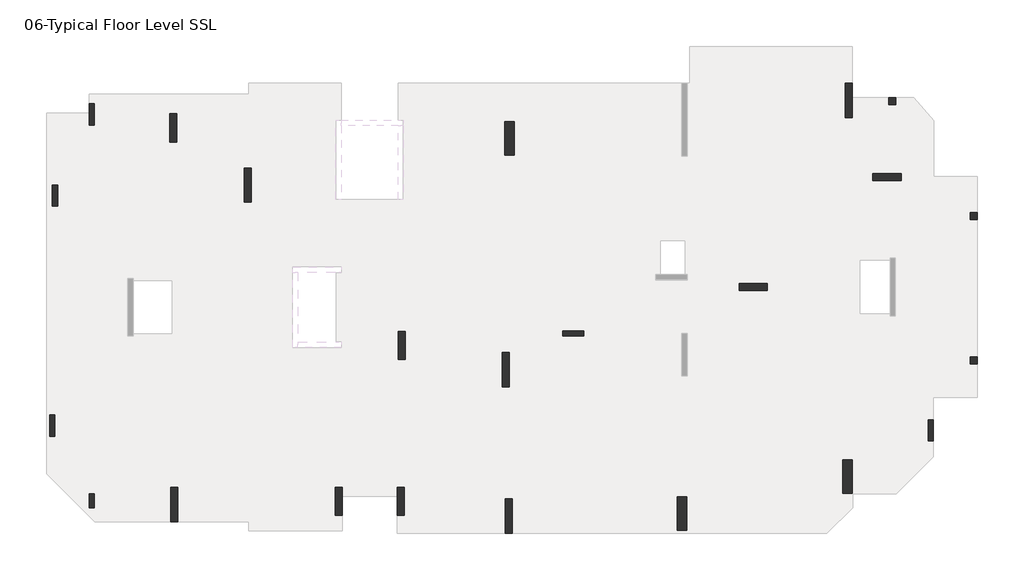
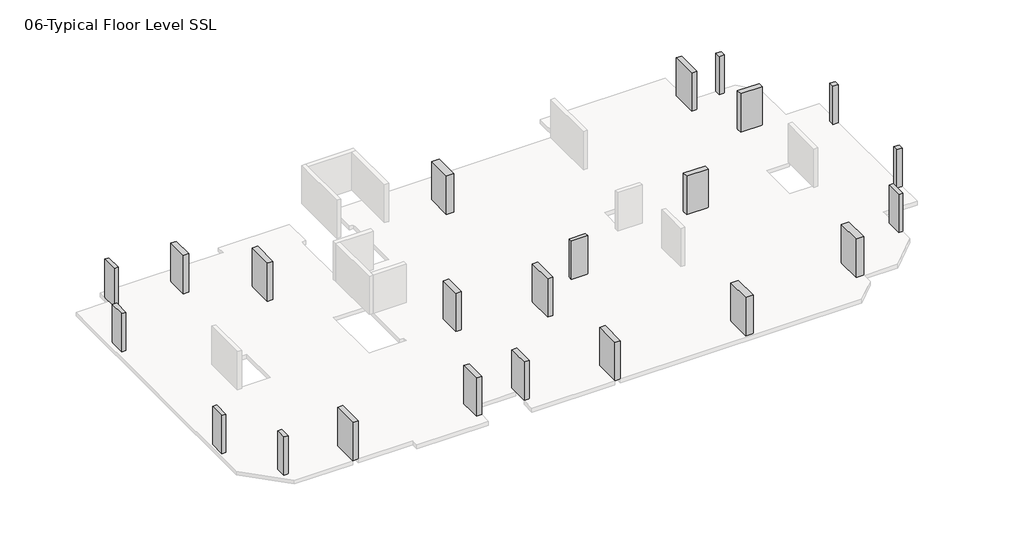
# One storey, part 2 of 2: 23 columns.
"""IFC4 building model written with IfcOpenShell, lengths in millimetres."""

import ifcopenshell
import ifcopenshell.guid

model = None  # the IFC model being written
_history = None  # IfcOwnerHistory: only IFC2X3 demands one
_inside = {}  # id of a spatial element -> (the spatial element, [elements in it])
_under = {}  # id of a project, library or spatial element -> (it, [spatial elements below it])
_declared = {}  # id of a project -> (the project, [libraries it declares])
_typed = {}  # id of a type object -> (the type object, [elements of that type])
_made_of = {}  # id of a material, layer set ... -> (it, [elements and type objects made of it])


def new_model(schema):
    """Start an empty IFC model of exactly this schema.

    Asked for "IFC4X3", IfcOpenShell would pick the latest addendum, in which some entities
    have other attributes; the version numbers below select the first issue.
    IFC2X3 requires an IfcOwnerHistory on every rooted entity: one is made here for all.
    """
    global model, _history
    if schema == "IFC4X3":
        model = ifcopenshell.file(schema_version=(4, 3, 0, 0))
    else:
        model = ifcopenshell.file(schema=schema)
    _inside.clear()
    _under.clear()
    _declared.clear()
    _typed.clear()
    _made_of.clear()
    _history = None
    if model.schema == "IFC2X3":
        org = make("IfcOrganization", Name="unknown")
        user = make(
            "IfcPersonAndOrganization",
            ThePerson=make("IfcPerson", FamilyName="unknown"),
            TheOrganization=org,
        )
        app = make(
            "IfcApplication",
            ApplicationDeveloper=org,
            Version="unknown",
            ApplicationFullName="unknown",
            ApplicationIdentifier="unknown",
        )
        _history = make(
            "IfcOwnerHistory",
            OwningUser=user,
            OwningApplication=app,
            ChangeAction="ADDED",
            CreationDate=0,
        )
    return model


def make(cls, **values):
    """One entity of the class cls with the attributes given. An attribute that is None is left unset."""
    return model.create_entity(
        cls, **{name: value for name, value in values.items() if value is not None}
    )


def rooted(cls, **values):
    """An entity with a GlobalId (a new one), such as an element, a storey or a relation."""
    return make(cls, GlobalId=ifcopenshell.guid.new(), OwnerHistory=_history, **values)


def si_unit(unit_type, name, prefix=None):
    """IfcSIUnit, for example si_unit("LENGTHUNIT", "METRE", prefix="MILLI")."""
    return make("IfcSIUnit", UnitType=unit_type, Prefix=prefix, Name=name)


def assignment(units):
    """IfcUnitAssignment: the units of a project."""
    return None if units is None else make("IfcUnitAssignment", Units=units)


def point(xyz):
    """IfcCartesianPoint."""
    return None if xyz is None else make("IfcCartesianPoint", Coordinates=xyz)


def direction(xyz):
    """IfcDirection."""
    return None if xyz is None else make("IfcDirection", DirectionRatios=xyz)


def frame(location, z_axis=None, x_axis=None):
    """IfcAxis2Placement3D, a coordinate frame: its origin and axes. An axis left out is left unset."""
    return make(
        "IfcAxis2Placement3D",
        Location=point(location),
        Axis=direction(z_axis),
        RefDirection=direction(x_axis),
    )


def origin():
    """The frame at (0, 0, 0) with its axes left unset."""
    return frame((0.0, 0.0, 0.0))


def place(relative_to, where):
    """IfcLocalPlacement: puts the frame where relative to a parent placement (None: the world)."""
    return make(
        "IfcLocalPlacement", PlacementRelTo=relative_to, RelativePlacement=where
    )


def context(
    kind, dimensions, precision=None, world=None, true_north=None, identifier=None
):
    """IfcGeometricRepresentationContext, for example the 3D "Model" context."""
    return make(
        "IfcGeometricRepresentationContext",
        ContextIdentifier=identifier,
        ContextType=kind,
        CoordinateSpaceDimension=dimensions,
        Precision=precision,
        WorldCoordinateSystem=world,
        TrueNorth=true_north,
    )


def project(units=None, contexts=None):
    """IfcProject with its units and contexts."""
    return rooted(
        "IfcProject",
        Name="project",
        RepresentationContexts=contexts,
        UnitsInContext=assignment(units),
    )


def spatial(cls, under=None, at=None, **own):
    """A site, building, storey or space (cls), placed at a placement, below another one or the project."""
    s = rooted(cls, ObjectPlacement=at, **own)
    if under is not None:
        _under.setdefault(under.id(), (under, []))[1].append(s)
    return s


def faces_of(points, faces, orient=None, outer=None):
    """IfcFace entities. A face is a list of loops; a loop is a list of indices into points, from 0.

    orient and outer hold one flag for each loop. By default every Orientation is true, the
    first loop of a face is its IfcFaceOuterBound and the others are IfcFaceBound.
    """
    made = []
    for i, loops in enumerate(faces):
        bounds = []
        for j, loop in enumerate(loops):
            is_outer = j == 0 if outer is None else outer[i][j]
            bounds.append(
                make(
                    "IfcFaceOuterBound" if is_outer else "IfcFaceBound",
                    Bound=make("IfcPolyLoop", Polygon=[points[k] for k in loop]),
                    Orientation=True if orient is None else orient[i][j],
                )
            )
        made.append(make("IfcFace", Bounds=bounds))
    return made


def faceted_brep(points, faces, orient=None, outer=None, voids=None):
    """IfcFacetedBrep: a solid bounded by flat faces; with voids (closed shells), ...WithVoids."""
    shared = [point(p) for p in points]
    hull = make("IfcClosedShell", CfsFaces=faces_of(shared, faces, orient, outer))
    if voids is None:
        return make("IfcFacetedBrep", Outer=hull)
    return make(
        "IfcFacetedBrepWithVoids",
        Outer=hull,
        Voids=[
            make(cls, CfsFaces=faces_of(shared, fs, o, b)) for cls, fs, o, b in voids
        ],
    )


def shape(context_of_items, identifier, shape_type, items):
    """IfcShapeRepresentation: the items that make up one representation, for example the "Body"."""
    return make(
        "IfcShapeRepresentation",
        ContextOfItems=context_of_items,
        RepresentationIdentifier=identifier,
        RepresentationType=shape_type,
        Items=items,
    )


def made_of(thing, what):
    """Note that an element or type object is made of a material, layer set ...; save() writes the relation."""
    if what is not None:
        _made_of.setdefault(what.id(), (what, []))[1].append(thing)
    return thing


def element(
    cls,
    number,
    at=None,
    inside=None,
    cuts=None,
    type_object=None,
    material=None,
    context=None,
    identifier="Body",
    shape_type=None,
    held_by="IfcProductDefinitionShape",
    body=None,
    shapes=None,
    **own,
):
    """One element of the class cls, such as IfcWall. Its Tag is "e" and its number.

    at: its placement. inside: the storey or other place that contains it. cuts: it is an
    opening in that element (IfcRelVoidsElement). A single representation is given by context,
    identifier, shape_type and body (its items); several are given by shapes. held_by: the class
    of the entity that holds the representations. save() writes the other relations.
    """
    e = rooted(cls, Tag="e%d" % number, ObjectPlacement=at, **own)
    if body is not None:
        shapes = [shape(context, identifier, shape_type, body)]
    if shapes is not None:
        e.Representation = make(held_by, Representations=shapes)
    if inside is not None:
        _inside.setdefault(inside.id(), (inside, []))[1].append(e)
    if cuts is not None:
        rooted(
            "IfcRelVoidsElement", RelatingBuildingElement=cuts, RelatedOpeningElement=e
        )
    if type_object is not None:
        _typed.setdefault(type_object.id(), (type_object, []))[1].append(e)
    return made_of(e, material)


def aggregate(whole, parts):
    """IfcRelAggregates: a whole, such as a stair, and the parts it consists of."""
    return rooted("IfcRelAggregates", RelatingObject=whole, RelatedObjects=parts)


def save(model, path):
    """Write the relations noted so far, then the file.

    IfcRelAggregates (storeys below a building ...), IfcRelContainedInSpatialStructure (elements
    in a storey), IfcRelDefinesByType, IfcRelAssociatesMaterial and IfcRelDeclares: one each for
    every whole, place, type object, material and project.
    """
    for whole, parts in _under.values():
        aggregate(whole, parts)
    for where, things in _inside.values():
        rooted(
            "IfcRelContainedInSpatialStructure",
            RelatedElements=things,
            RelatingStructure=where,
        )
    for kind, things in _typed.values():
        rooted("IfcRelDefinesByType", RelatedObjects=things, RelatingType=kind)
    for what, things in _made_of.values():
        rooted("IfcRelAssociatesMaterial", RelatedObjects=things, RelatingMaterial=what)
    for by, libraries in _declared.values():
        rooted("IfcRelDeclares", RelatingContext=by, RelatedDefinitions=libraries)
    model.write(path)


model = new_model("IFC4")

# Units and contexts
model_context = context("Model", 3, world=origin())
ifc_project = project(units=[si_unit("LENGTHUNIT", "METRE", prefix="MILLI")], contexts=[model_context])

# Site, building, storey
site = spatial("IfcSite", under=ifc_project)
building = spatial("IfcBuilding", under=site)
storey = spatial("IfcBuildingStorey", under=building, Name="06-Typical Floor Level SSL", Elevation=12000.0)

# Columns
placement = place(None, origin())
element("IfcColumn", 1, ObjectType="M_Concrete-Rectangular-Column : C-1 (400 x 400mm)", at=placement, inside=storey, context=model_context, shape_type="Brep", body=[
    faceted_brep([(52549.9999998, 16712.0, 12000.0), (52549.9999998, 16312.0, 12000.0), (52149.9999998, 16312.0, 12000.0), (52149.9999998, 16712.0, 12000.0), (52549.9999998, 16712.0, 15000.0), (52549.9999998, 16312.0, 15000.0), (52549.9999998, 16312.0, 14700.0), (52549.9999998, 16712.0, 14700.0), (52149.9999998, 16312.0, 15000.0), (52149.9999998, 16312.0, 14700.0), (52149.9999998, 16712.0, 15000.0), (52149.9999998, 16712.0, 14700.0)], [[[0, 1, 2, 3]], [[4, 5, 6, 1, 0, 7]], [[5, 8, 9, 2, 1, 6]], [[8, 10, 11, 3, 2, 9]], [[10, 4, 7, 0, 3, 11]], [[4, 10, 8, 5]]]),
])
element("IfcColumn", 2, ObjectType="M_Concrete-Rectangular-Column : C-1 (400 x 400mm)", at=placement, inside=storey, context=model_context, shape_type="Brep", body=[
    faceted_brep([(47898.6337868, 23252.0, 12000.0), (47898.6337868, 22852.0, 12000.0), (47498.6337868, 22852.0, 12000.0), (47498.6337868, 23252.0, 12000.0), (47898.6337868, 23252.0, 15000.0), (47898.6337868, 22852.0, 15000.0), (47898.6337868, 22852.0, 14700.0), (47498.6337868, 22852.0, 15000.0), (47498.6337868, 22852.0, 14700.0), (47498.6337868, 23252.0, 15000.0)], [[[0, 1, 2, 3]], [[4, 5, 6, 1, 0]], [[5, 7, 8, 2, 1, 6]], [[7, 9, 3, 2, 8]], [[9, 4, 0, 3]], [[4, 9, 7, 5]]]),
])
element("IfcColumn", 3, ObjectType="M_Concrete-Rectangular-Column : C-1 (400 x 400mm)", at=placement, inside=storey, context=model_context, shape_type="Brep", body=[
    faceted_brep([(52549.9999998, 8504.0039609, 12000.0), (52549.9999998, 8104.0039609, 12000.0), (52149.9999998, 8104.0039609, 12000.0), (52149.9999998, 8504.0039609, 12000.0), (52549.9999998, 8504.0039609, 15000.0), (52549.9999998, 8104.0039609, 15000.0), (52549.9999998, 8104.0039609, 14700.0), (52549.9999998, 8504.0039609, 14700.0), (52149.9999998, 8104.0039609, 15000.0), (52149.9999998, 8104.0039609, 14700.0), (52149.9999998, 8504.0039609, 15000.0), (52149.9999998, 8504.0039609, 14700.0)], [[[0, 1, 2, 3]], [[4, 5, 6, 1, 0, 7]], [[5, 8, 9, 2, 1, 6]], [[8, 10, 11, 3, 2, 9]], [[10, 4, 7, 0, 3, 11]], [[4, 10, 8, 5]]]),
])
element("IfcColumn", 4, ObjectType="M_Concrete-Rectangular-Column : C-2 (300 x 800mm)", at=placement, inside=storey, context=model_context, shape_type="Brep", body=[
    faceted_brep([(2352.0, 728.0, 12000.0), (2352.0, -72.0, 12000.0), (2052.0, -72.0, 12000.0), (2052.0, 728.0, 12000.0), (2352.0, 728.0, 15000.0), (2352.0, -72.0, 15000.0), (2352.0, -72.0, 14700.0), (2352.0, 728.0, 14700.0), (2052.0, -72.0, 15000.0), (2052.0, -72.0, 14700.0), (2052.0, 728.0, 15000.0), (2052.0, 728.0, 14700.0)], [[[0, 1, 2, 3]], [[4, 5, 6, 1, 0, 7]], [[5, 8, 9, 2, 1, 6]], [[8, 10, 11, 3, 2, 9]], [[10, 4, 7, 0, 3, 11]], [[4, 10, 8, 5]]]),
])
element("IfcColumn", 5, ObjectType="M_Concrete-Rectangular-Column : C-3(300 x 1200mm)", at=placement, inside=storey, context=model_context, shape_type="Brep", body=[
    faceted_brep([(2352.0, 22908.0000656, 12000.0), (2352.0, 21708.0000656, 12000.0), (2052.0, 21708.0000656, 12000.0), (2052.0, 22908.0000656, 12000.0), (2352.0, 22908.0000656, 15000.0), (2352.0, 21708.0000656, 15000.0), (2352.0, 21708.0000656, 14700.0), (2352.0, 22908.0000656, 14700.0), (2052.0, 21708.0000656, 15000.0), (2052.0, 21708.0000656, 14700.0), (2052.0, 22380.0004589, 15000.0), (2052.0, 22908.0000656, 15000.0), (2052.0, 22908.0000656, 14700.0)], [[[0, 1, 2, 3]], [[4, 5, 6, 1, 0, 7]], [[5, 8, 9, 2, 1, 6]], [[8, 10, 11, 12, 3, 2, 9]], [[11, 4, 7, 0, 3, 12]], [[4, 11, 10, 8, 5]]]),
])
element("IfcColumn", 6, ObjectType="M_Concrete-Rectangular-Column : C-3(300 x 1200mm)", at=placement, inside=storey, context=model_context, shape_type="Brep", body=[
    faceted_brep([(257.9999999, 18288.0, 12000.0), (257.9999999, 17088.0, 12000.0), (-42.0000001, 17088.0, 12000.0), (-42.0000001, 18288.0, 12000.0), (257.9999999, 18288.0, 15000.0), (257.9999999, 17088.0, 15000.0), (257.9999999, 17088.0, 14700.0), (257.9999999, 18288.0, 14700.0), (-42.0000001, 17088.0, 15000.0), (-42.0000001, 17088.0, 14700.0), (-42.0000001, 18288.0, 15000.0), (-42.0000001, 18288.0, 14700.0)], [[[0, 1, 2, 3]], [[4, 5, 6, 1, 0, 7]], [[5, 8, 9, 2, 1, 6]], [[8, 10, 11, 3, 2, 9]], [[10, 4, 7, 0, 3, 11]], [[4, 10, 8, 5]]]),
])
element("IfcColumn", 7, ObjectType="M_Concrete-Rectangular-Column : C-3(300 x 1200mm)", at=placement, inside=storey, context=model_context, shape_type="Brep", body=[
    faceted_brep([(108.001803, 5201.9999858, 12000.0), (108.001803, 4001.9999858, 12000.0), (-191.998197, 4001.9999858, 12000.0), (-191.998197, 5201.9999858, 12000.0), (108.001803, 5201.9999858, 15000.0), (108.001803, 4001.9999858, 15000.0), (108.001803, 4001.9999858, 14700.0), (108.001803, 5201.9999858, 14700.0), (-191.998197, 4001.9999858, 15000.0), (-191.998197, 4001.9999858, 14700.0), (-191.998197, 5201.9999858, 15000.0), (-191.998197, 5201.9999858, 14700.0)], [[[0, 1, 2, 3]], [[4, 5, 6, 1, 0, 7]], [[5, 8, 9, 2, 1, 6]], [[8, 10, 11, 3, 2, 9]], [[10, 4, 7, 0, 3, 11]], [[4, 10, 8, 5]]]),
])
element("IfcColumn", 8, ObjectType="M_Concrete-Rectangular-Column : C-3(300 x 1200mm)", at=placement, inside=storey, context=model_context, shape_type="Brep", body=[
    faceted_brep([(50046.0009271, 4931.9999929, 12000.0), (50046.0009271, 3731.9999929, 12000.0), (49746.0009271, 3731.9999929, 12000.0), (49746.0009271, 4931.9999929, 12000.0), (50046.0009271, 4931.9999929, 15000.0), (50046.0009271, 3731.9999929, 15000.0), (50046.0009271, 3731.9999929, 14700.0), (50046.0009271, 4931.9999929, 14700.0), (49746.0009271, 3731.9999929, 15000.0), (49746.0009271, 3731.9999929, 14700.0), (49746.0009271, 4931.9999929, 15000.0), (49746.0009271, 4931.9999929, 14700.0)], [[[0, 1, 2, 3]], [[4, 5, 6, 1, 0, 7]], [[5, 8, 9, 2, 1, 6]], [[8, 10, 11, 3, 2, 9]], [[10, 4, 7, 0, 3, 11]], [[4, 10, 8, 5]]]),
])
element("IfcColumn", 9, ObjectType="M_Concrete-Rectangular-Column : C-3(300 x 1200mm)", at=placement, inside=storey, context=model_context, shape_type="Brep", body=[
    faceted_brep([(28975.9999998, 9996.0000019, 12000.0), (30175.9999998, 9996.0000019, 12000.0), (30175.9999998, 9696.0000019, 12000.0), (28975.9999998, 9696.0000019, 12000.0), (28975.9999998, 9996.0000019, 15000.0), (30175.9999998, 9996.0000019, 15000.0), (30175.9999998, 9996.0000019, 14700.0), (28975.9999998, 9996.0000019, 14700.0), (30175.9999998, 9696.0000019, 15000.0), (30175.9999998, 9696.0000019, 14700.0), (28975.9999998, 9696.0000019, 15000.0), (28975.9999998, 9696.0000019, 14700.0)], [[[0, 1, 2, 3]], [[4, 5, 6, 1, 0, 7]], [[5, 8, 9, 2, 1, 6]], [[8, 10, 11, 3, 2, 9]], [[10, 4, 7, 0, 3, 11]], [[4, 10, 8, 5]]]),
])
element("IfcColumn", 10, ObjectType="M_Concrete-Rectangular-Column : C-4 (400 x 1600mm)", at=placement, inside=storey, context=model_context, shape_type="Brep", body=[
    faceted_brep([(7021.9999999, 22340.0000078, 12000.0), (7021.9999999, 20740.0000078, 12000.0), (6621.9999999, 20740.0000078, 12000.0), (6621.9999999, 22340.0000078, 12000.0), (7021.9999999, 22340.0000078, 15000.0), (7021.9999999, 20740.0000078, 15000.0), (7021.9999999, 20740.0000078, 14700.0), (7021.9999999, 22340.0000078, 14700.0), (6621.9999999, 20740.0000078, 15000.0), (6621.9999999, 20740.0000078, 14700.0), (6621.9999999, 22340.0000078, 15000.0), (6621.9999999, 22340.0000078, 14700.0)], [[[0, 1, 2, 3]], [[4, 5, 6, 1, 0, 7]], [[5, 8, 9, 2, 1, 6]], [[8, 10, 11, 3, 2, 9]], [[10, 4, 7, 0, 3, 11]], [[4, 10, 8, 5]]]),
])
element("IfcColumn", 11, ObjectType="M_Concrete-Rectangular-Column : C-4 (400 x 1600mm)", at=placement, inside=storey, context=model_context, shape_type="Brep", body=[
    faceted_brep([(19969.9997488, 1087.9955348, 12000.0), (19969.9997488, -512.0044652, 12000.0), (19569.9997488, -512.0044652, 12000.0), (19569.9997488, 1087.9955348, 12000.0), (19969.9997488, 1087.9955348, 15000.0), (19969.9997488, -512.0044652, 15000.0), (19969.9997488, -512.0044652, 14700.0), (19969.9997488, 1087.9955348, 14700.0), (19569.9997488, -512.0044652, 15000.0), (19569.9997488, -512.0044652, 14700.0), (19569.9997488, 564.000519, 15000.0), (19569.9997488, 1087.9955348, 15000.0), (19569.9997488, 1087.9955348, 14700.0)], [[[0, 1, 2, 3]], [[4, 5, 6, 1, 0, 7]], [[5, 8, 9, 2, 1, 6]], [[8, 10, 11, 12, 3, 2, 9]], [[11, 4, 7, 0, 3, 12]], [[4, 11, 10, 8, 5]]]),
])
element("IfcColumn", 12, ObjectType="M_Concrete-Rectangular-Column : C-4 (400 x 1600mm)", at=placement, inside=storey, context=model_context, shape_type="Brep", body=[
    faceted_brep([(46605.9993605, 18950.0, 12000.0), (48205.9993605, 18950.0, 12000.0), (48205.9993605, 18550.0, 12000.0), (46605.9993605, 18550.0, 12000.0), (46605.9993605, 18950.0, 15000.0), (48205.9993605, 18950.0, 15000.0), (48205.9993605, 18950.0, 14700.0), (46605.9993605, 18950.0, 14700.0), (48205.9993605, 18550.0, 15000.0), (48205.9993605, 18550.0, 14700.0), (46605.9993605, 18550.0, 15000.0), (46605.9993605, 18550.0, 14700.0)], [[[0, 1, 2, 3]], [[4, 5, 6, 1, 0, 7]], [[5, 8, 9, 2, 1, 6]], [[8, 10, 11, 3, 2, 9]], [[10, 4, 7, 0, 3, 11]], [[4, 10, 8, 5]]]),
])
element("IfcColumn", 13, ObjectType="M_Concrete-Rectangular-Column : C-5 (400 x 1600mm)", at=placement, inside=storey, context=model_context, shape_type="Brep", body=[
    faceted_brep([(20030.000009, 9955.9999979, 12000.0), (20030.000009, 8355.9999979, 12000.0), (19630.000009, 8355.9999979, 12000.0), (19630.000009, 9955.9999979, 12000.0), (20030.000009, 9955.9999979, 15000.0), (20030.000009, 8355.9999979, 15000.0), (20030.000009, 8355.9999979, 14700.0), (20030.000009, 9955.9999979, 14700.0), (19630.000009, 8355.9999979, 15000.0), (19630.000009, 8355.9999979, 14700.0), (19630.000009, 9955.9999979, 15000.0), (19630.000009, 9955.9999979, 14700.0)], [[[0, 1, 2, 3]], [[4, 5, 6, 1, 0, 7]], [[5, 8, 9, 2, 1, 6]], [[8, 10, 11, 3, 2, 9]], [[10, 4, 7, 0, 3, 11]], [[4, 10, 8, 5]]]),
])
element("IfcColumn", 14, ObjectType="M_Concrete-Rectangular-Column : C-5 (400 x 1600mm)", at=placement, inside=storey, context=model_context, shape_type="Brep", body=[
    faceted_brep([(16429.9999981, 1088.0, 12000.0), (16429.9999981, -512.0, 12000.0), (16029.9999981, -512.0, 12000.0), (16029.9999981, 1088.0, 12000.0), (16429.9999981, 1088.0, 15000.0), (16429.9999981, 564.000519, 15000.0), (16429.9999981, -512.0, 15000.0), (16429.9999981, -512.0, 14700.0), (16429.9999981, 1088.0, 14700.0), (16029.9999981, -512.0, 15000.0), (16029.9999981, -512.0, 14700.0), (16029.9999981, 1088.0, 15000.0), (16029.9999981, 1088.0, 14700.0)], [[[0, 1, 2, 3]], [[4, 5, 6, 7, 1, 0, 8]], [[6, 9, 10, 2, 1, 7]], [[9, 11, 12, 3, 2, 10]], [[11, 4, 8, 0, 3, 12]], [[4, 11, 9, 6, 5]]]),
])
element("IfcColumn", 15, ObjectType="M_Concrete-Rectangular-Column : C-5 (400 x 1600mm)", at=placement, inside=storey, context=model_context, shape_type="Brep", body=[
    faceted_brep([(38998.0014887, 12692.0079212, 12000.0), (40598.0014887, 12692.0079212, 12000.0), (40598.0014887, 12292.0079212, 12000.0), (38998.0014887, 12292.0079212, 12000.0), (38998.0014887, 12692.0079212, 15000.0), (40598.0014887, 12692.0079212, 15000.0), (40598.0014887, 12692.0079212, 14700.0), (38998.0014887, 12692.0079212, 14700.0), (40598.0014887, 12292.0079212, 15000.0), (40598.0014887, 12292.0079212, 14700.0), (38998.0014887, 12292.0079212, 15000.0), (38998.0014887, 12292.0079212, 14700.0)], [[[0, 1, 2, 3]], [[4, 5, 6, 1, 0, 7]], [[5, 8, 9, 2, 1, 6]], [[8, 10, 11, 3, 2, 9]], [[10, 4, 7, 0, 3, 11]], [[4, 10, 8, 5]]]),
])
element("IfcColumn", 16, ObjectType="M_Concrete-Rectangular-Column : C-6 (400 x 1950mm)", at=placement, inside=storey, context=model_context, shape_type="Brep", body=[
    faceted_brep([(11270.0000427, 19262.9999996, 12000.0), (11270.0000427, 17312.9999996, 12000.0), (10870.0000427, 17312.9999996, 12000.0), (10870.0000427, 19262.9999996, 12000.0), (11270.0000427, 19262.9999996, 15000.0), (11270.0000427, 17312.9999996, 15000.0), (11270.0000427, 17312.9999996, 14700.0), (11270.0000427, 19262.9999996, 14700.0), (10870.0000427, 17312.9999996, 15000.0), (10870.0000427, 17312.9999996, 14700.0), (10870.0000427, 19262.9999996, 15000.0), (10870.0000427, 19262.9999996, 14700.0)], [[[0, 1, 2, 3]], [[4, 5, 6, 1, 0, 7]], [[5, 8, 9, 2, 1, 6]], [[8, 10, 11, 3, 2, 9]], [[10, 4, 7, 0, 3, 11]], [[4, 10, 8, 5]]]),
])
element("IfcColumn", 17, ObjectType="M_Concrete-Rectangular-Column : C-6 (400 x 1950mm)", at=placement, inside=storey, context=model_context, shape_type="Brep", body=[
    faceted_brep([(7082.0000416, 1083.0000153, 12000.0), (7082.0000416, -866.9999847, 12000.0), (6682.0000416, -866.9999847, 12000.0), (6682.0000416, 1083.0000153, 12000.0), (7082.0000416, 1083.0000153, 15000.0), (7082.0000416, -866.9999847, 15000.0), (7082.0000416, -866.9999847, 14700.0), (7082.0000416, 1083.0000153, 14700.0), (6682.0000416, -866.9999847, 15000.0), (6682.0000416, -866.9999847, 14700.0), (6682.0000416, 1083.0000153, 15000.0), (6682.0000416, 1083.0000153, 14700.0)], [[[0, 1, 2, 3]], [[4, 5, 6, 1, 0, 7]], [[5, 8, 9, 2, 1, 6]], [[8, 10, 11, 3, 2, 9]], [[10, 4, 7, 0, 3, 11]], [[4, 10, 8, 5]]]),
])
element("IfcColumn", 18, ObjectType="M_Concrete-Rectangular-Column : C-6 (400 x 1950mm)", at=placement, inside=storey, context=model_context, shape_type="Brep", body=[
    faceted_brep([(26113.9999998, 422.995535, 12000.0), (26113.9999998, -1527.004465, 12000.0), (25713.9999998, -1527.004465, 12000.0), (25713.9999998, 422.995535, 12000.0), (26113.9999998, 422.995535, 15000.0), (26113.9999998, -1527.004465, 15000.0), (26113.9999998, -1527.004465, 14700.0), (26113.9999998, 422.995535, 14700.0), (25713.9999998, -1527.004465, 15000.0), (25713.9999998, -1527.004465, 14700.0), (25713.9999998, 422.995535, 15000.0), (25713.9999998, 422.995535, 14700.0)], [[[0, 1, 2, 3]], [[4, 5, 6, 1, 0, 7]], [[5, 8, 9, 2, 1, 6]], [[8, 10, 11, 3, 2, 9]], [[10, 4, 7, 0, 3, 11]], [[4, 10, 8, 5]]]),
])
element("IfcColumn", 19, ObjectType="M_Concrete-Rectangular-Column : C-6 (400 x 1950mm)", at=placement, inside=storey, context=model_context, shape_type="Brep", body=[
    faceted_brep([(45446.0007483, 24087.0, 12000.0), (45446.0007483, 22137.0, 12000.0), (45046.0007483, 22137.0, 12000.0), (45046.0007483, 24087.0, 12000.0), (45446.0007483, 24087.0, 15000.0), (45446.0007483, 23252.0000315, 15000.0), (45446.0007483, 22137.0, 15000.0), (45446.0007483, 22137.0, 14700.0), (45446.0007483, 24087.0, 14700.0), (45046.0007483, 22137.0, 15000.0), (45046.0007483, 22137.0, 14700.0), (45046.0007483, 24087.0, 15000.0), (45046.0007483, 24087.0, 14700.0)], [[[0, 1, 2, 3]], [[4, 5, 6, 7, 1, 0, 8]], [[6, 9, 10, 2, 1, 7]], [[9, 11, 12, 3, 2, 10]], [[11, 4, 8, 0, 3, 12]], [[4, 11, 9, 6, 5]]]),
])
element("IfcColumn", 20, ObjectType="M_Concrete-Rectangular-Column : C-6 (400 x 1950mm)", at=placement, inside=storey, context=model_context, shape_type="Brep", body=[
    faceted_brep([(25934.0000455, 8751.0001824, 12000.0), (25934.0000455, 6801.0001824, 12000.0), (25534.0000455, 6801.0001824, 12000.0), (25534.0000455, 8751.0001824, 12000.0), (25934.0000455, 8751.0001824, 15000.0), (25934.0000455, 6801.0001824, 15000.0), (25934.0000455, 6801.0001824, 14700.0), (25934.0000455, 8751.0001824, 14700.0), (25534.0000455, 6801.0001824, 15000.0), (25534.0000455, 6801.0001824, 14700.0), (25534.0000455, 8751.0001824, 15000.0), (25534.0000455, 8751.0001824, 14700.0)], [[[0, 1, 2, 3]], [[4, 5, 6, 1, 0, 7]], [[5, 8, 9, 2, 1, 6]], [[8, 10, 11, 3, 2, 9]], [[10, 4, 7, 0, 3, 11]], [[4, 10, 8, 5]]]),
])
element("IfcColumn", 21, ObjectType="M_Concrete-Rectangular-Column : C-7 (550 x 1900mm)", at=placement, inside=storey, context=model_context, shape_type="Brep", body=[
    faceted_brep([(36035.9999998, 548.0007983, 12000.0), (36035.9999998, -1351.9992017, 12000.0), (35485.9999998, -1351.9992017, 12000.0), (35485.9999998, 548.0007983, 12000.0), (36035.9999998, 548.0007983, 15000.0), (36035.9999998, -1351.9992017, 15000.0), (36035.9999998, -1351.9992017, 14700.0), (36035.9999998, 548.0007983, 14700.0), (35485.9999998, -1351.9992017, 15000.0), (35485.9999998, -1351.9992017, 14700.0), (35485.9999998, 548.0007983, 15000.0), (35485.9999998, 548.0007983, 14700.0)], [[[0, 1, 2, 3]], [[4, 5, 6, 1, 0, 7]], [[5, 8, 9, 2, 1, 6]], [[8, 10, 11, 3, 2, 9]], [[10, 4, 7, 0, 3, 11]], [[4, 10, 8, 5]]]),
])
element("IfcColumn", 22, ObjectType="M_Concrete-Rectangular-Column : C-7 (550 x 1900mm)", at=placement, inside=storey, context=model_context, shape_type="Brep", body=[
    faceted_brep([(45443.9999998, 2648.0, 12000.0), (45443.9999998, 748.0, 12000.0), (44893.9999998, 748.0, 12000.0), (44893.9999998, 2648.0, 12000.0), (45443.9999998, 2648.0, 15000.0), (45443.9999998, 748.0, 15000.0), (45443.9999998, 748.0, 14700.0), (45443.9999998, 2648.0, 14700.0), (44893.9999998, 748.0, 15000.0), (44893.9999998, 748.0, 14700.0), (44893.9999998, 2648.0, 15000.0), (44893.9999998, 2648.0, 14700.0)], [[[0, 1, 2, 3]], [[4, 5, 6, 1, 0, 7]], [[5, 8, 9, 2, 1, 6]], [[8, 10, 11, 3, 2, 9]], [[10, 4, 7, 0, 3, 11]], [[4, 10, 8, 5]]]),
])
element("IfcColumn", 23, ObjectType="M_Concrete-Rectangular-Column : C-7 (550 x 1900mm)", at=placement, inside=storey, context=model_context, shape_type="Brep", body=[
    faceted_brep([(26218.9999998, 21900.0, 12000.0), (26218.9999998, 20000.0, 12000.0), (25668.9999998, 20000.0, 12000.0), (25668.9999998, 21900.0, 12000.0), (26218.9999998, 21900.0, 15000.0), (26218.9999998, 20000.0, 15000.0), (26218.9999998, 20000.0, 14700.0), (26218.9999998, 21900.0, 14700.0), (25668.9999998, 20000.0, 15000.0), (25668.9999998, 20000.0, 14700.0), (25668.9999998, 21900.0, 15000.0), (25668.9999998, 21900.0, 14700.0)], [[[0, 1, 2, 3]], [[4, 5, 6, 1, 0, 7]], [[5, 8, 9, 2, 1, 6]], [[8, 10, 11, 3, 2, 9]], [[10, 4, 7, 0, 3, 11]], [[4, 10, 8, 5]]]),
])

save(model, "model.ifc")

# Revit data of these elements
# Type "M_Concrete-Rectangular-Column : C-1 (400 x 400mm)"
#   Type Mark = "C01"
#   b = 400 mm
#   h = 400 mm
#   Structural Material [instance default] = Concrete, Cast-in-Place gray
# Type "M_Concrete-Rectangular-Column : C-2 (300 x 800mm)"
#   Type Mark = "C02"
#   b = 300 mm
#   h = 800 mm
#   Structural Material [instance default] = Concrete, Cast-in-Place gray
# Type "M_Concrete-Rectangular-Column : C-3(300 x 1200mm)"
#   Type Mark = "C03"
#   b = 300 mm
#   h = 1200 mm
#   Structural Material [instance default] = Concrete, Cast-in-Place gray
# Type "M_Concrete-Rectangular-Column : C-4 (400 x 1600mm)"
#   Type Mark = "C04"
#   b = 400 mm
#   h = 1600 mm
#   Structural Material [instance default] = Concrete, Cast-in-Place gray
# Type "M_Concrete-Rectangular-Column : C-5 (400 x 1600mm)"
#   Type Mark = "C05"
#   b = 400 mm
#   h = 1600 mm
#   Structural Material [instance default] = Concrete, Cast-in-Place gray
# Type "M_Concrete-Rectangular-Column : C-6 (400 x 1950mm)"
#   Type Mark = "C06"
#   b = 400 mm
#   h = 1950 mm
#   Structural Material [instance default] = Concrete, Cast-in-Place gray
# Type "M_Concrete-Rectangular-Column : C-7 (550 x 1900mm)"
#   Type Mark = "C07"
#   b = 550 mm
#   h = 1900 mm
#   Structural Material [instance default] = Concrete, Cast-in-Place gray
# Elements 1, 2, 3 (IfcColumn, "M_Concrete-Rectangular-Column : C-1 (400 x 400mm)")
#   Structural Material = Concrete-RC
#   Phase Created = New Construction
#   Materials on its faces: "Concrete-RC"
# Element 4 (IfcColumn, "M_Concrete-Rectangular-Column : C-2 (300 x 800mm)")
#   Structural Material = Concrete-RC
#   Phase Created = New Construction
#   Materials on its faces: "Concrete-RC"
# Elements 5, 6, 7, 8, 9 (IfcColumn, "M_Concrete-Rectangular-Column : C-3(300 x 1200mm)")
#   Structural Material = Concrete-RC
#   Phase Created = New Construction
#   Materials on its faces: "Concrete-RC"
# Elements 10, 11, 12 (IfcColumn, "M_Concrete-Rectangular-Column : C-4 (400 x 1600mm)")
#   Structural Material = Concrete-RC
#   Phase Created = New Construction
#   Materials on its faces: "Concrete-RC"
# Elements 13, 14, 15 (IfcColumn, "M_Concrete-Rectangular-Column : C-5 (400 x 1600mm)")
#   Structural Material = Concrete-RC
#   Phase Created = New Construction
#   Materials on its faces: "Concrete-RC"
# Elements 16, 17, 18, 19, 20 (IfcColumn, "M_Concrete-Rectangular-Column : C-6 (400 x 1950mm)")
#   Structural Material = Concrete-RC
#   Phase Created = New Construction
#   Materials on its faces: "Concrete-RC"
# Elements 21, 22, 23 (IfcColumn, "M_Concrete-Rectangular-Column : C-7 (550 x 1900mm)")
#   Structural Material = Concrete-RC
#   Phase Created = New Construction
#   Materials on its faces: "Concrete-RC"
# Materials
#   "Concrete, Cast-in-Place gray": class "Concrete", colour RGB 192 192 192, transparency 0, Description = "Cast-in-place concrete", Cost = 0
#   "Concrete-RC": class "Concrete", colour RGB 128 128 128, transparency 0, Description = "High strength concrete", Cost = 0
